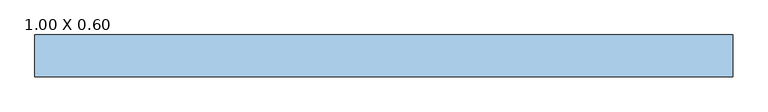
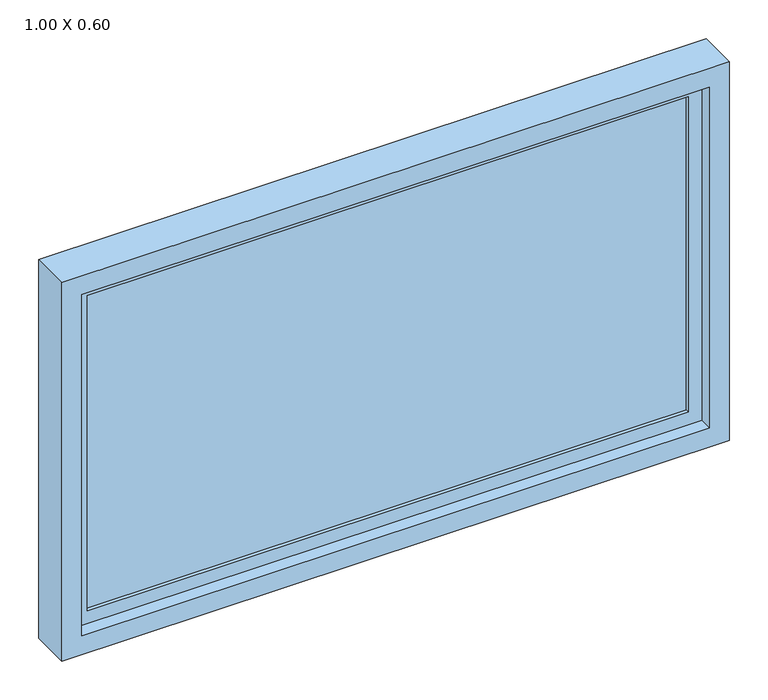
"""IFC4 building model written with IfcOpenShell, lengths in millimetres: window geometry, .CC_ND 300_MAXIM-AR : 1.00 X 0.60."""

from ifc_helpers import new_model, si_unit, frame, origin, place, context, project, spatial, polyline, outline, extrude, source, transform, mapped, element, save


def window_1_00_x_0_60_b9f016d9(model_context):
    return source(origin(), model_context, "Body", "SweptSolid", [
        extrude(outline(polyline([(-450.0, -4.0), (-450.0, 4.0), (450.0, 4.0), (450.0, -4.0), (-450.0, -4.0)])), frame((0.0, 0.0, 1550.0), z_axis=(0.0, 0.0, 1.0), x_axis=(1.0, 0.0, 0.0)), (0.0, 0.0, 1.0), 500.0),
        extrude(outline(polyline([(1530.0, 470.0), (2070.0, 470.0), (2070.0, -470.0), (1530.0, -470.0), (1530.0, 470.0)]), holes=[polyline([(2050.0, 450.0), (1550.0, 450.0), (1550.0, -450.0), (2050.0, -450.0), (2050.0, 450.0)])]), frame((0.0, -10.0, 0.0), z_axis=(0.0, 1.0, 0.0), x_axis=(0.0, 0.0, 1.0)), (0.0, 0.0, 1.0), 20.0),
        extrude(outline(polyline([(1500.0, 500.0), (2100.0, 500.0), (2100.0, -500.0), (1500.0, -500.0), (1500.0, 500.0)]), holes=[polyline([(2070.0, 470.0), (1530.0, 470.0), (1530.0, -470.0), (2070.0, -470.0), (2070.0, 470.0)])]), frame((0.0, -30.0, 0.0), z_axis=(0.0, 1.0, 0.0), x_axis=(0.0, 0.0, 1.0)), (0.0, 0.0, 1.0), 60.0),
    ])


if __name__ == "__main__":
    model = new_model("IFC4")
    model_context = context("Model", 3, world=origin())
    ifc_project = project(units=[si_unit("LENGTHUNIT", "METRE", prefix="MILLI")], contexts=[model_context])
    site = spatial("IfcSite", under=ifc_project)
    building = spatial("IfcBuilding", under=site)
    placement = place(None, origin())
    window_1_00_x_0_60_shape = window_1_00_x_0_60_b9f016d9(model_context)
    element("IfcWindow", 1, ObjectType=".CC_ND 300_MAXIM-AR : 1.00 X 0.60", at=placement, inside=building, context=model_context, shape_type="MappedRepresentation", body=[
        mapped(window_1_00_x_0_60_shape, transform((0.0, 0.0, 0.0), x_axis=(1.0, 0.0, 0.0), y_axis=(0.0, 1.0, 0.0), z_axis=(0.0, 0.0, 1.0))),
    ])
    save(model, "model.ifc")

# Revit data of these elements
# Type ".CC_ND 300_MAXIM-AR : 1.00 X 0.60"
#   Type Mark = "67"
#   Largura Painel [instance default] = 0.02 m
#   Largura Esquadria [instance default] = 0.06 m
#   Espessura Vidro [instance default] = 0.008 m
#   Espessura Painel [instance default] = 0.02 m
#   Espessura Esquadria [instance default] = 0.03 m
#   Height = 0.60 m
#   Altura-padrão do peitoril = 1.50 m
#   Width = 1.00 m
#   Vidro = .VIDRO GENÉRICO
#   Esquadria = .ALUMÍNIO COM PINTURA ELETROSTÁTICA BRANCA
#   Wall Closure = (empty or 0)
# Element 1 (IfcWindow, ".CC_ND 300_MAXIM-AR : 1.00 X 0.60")
#   Materials on its faces: ".ALUMÍNIO COM PINTURA ELETROSTÁTICA BRANCA", ".VIDRO GENÉRICO"
# Materials
#   ".VIDRO GENÉRICO": class ".CC_VIDRO", colour RGB 0 128 192, transparency 0.9, Description = "Vidro comum", Cost = 0
#   ".ALUMÍNIO COM PINTURA ELETROSTÁTICA BRANCA": class "CC_METAIS", colour RGB 241 241 241, transparency 0, Cost = 0
